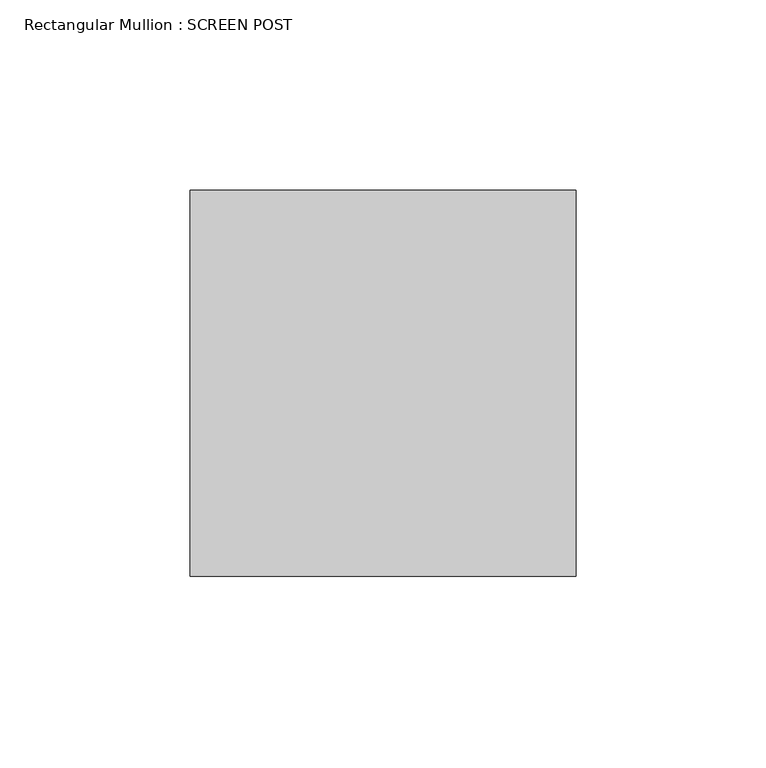
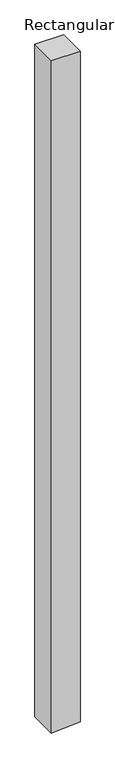
"""IFC4 building model written with IfcOpenShell, lengths in millimetres: member geometry, Rectangular Mullion : SCREEN POST."""

from ifc_helpers import new_model, si_unit, frame, origin, place, context, project, spatial, polyline, outline, extrude, source, transform, mapped, element, save


def rectangular_mullion_screen_post_f0368bff(model_context):
    return source(origin(), model_context, "Body", "SweptSolid", [
        extrude(outline(polyline([(0.0, 50.8), (0.0, -50.8), (-2524.2283574, -50.8), (-2521.4451532, -6.3490391), (-2517.8668852, 50.8), (0.0, 50.8)])), frame((0.0, -50.8, 0.0), z_axis=(0.0, 1.0, 0.0), x_axis=(0.0, 0.0, 1.0)), (0.0, 0.0, 1.0), 101.6),
    ])


if __name__ == "__main__":
    model = new_model("IFC4")
    model_context = context("Model", 3, world=origin())
    ifc_project = project(units=[si_unit("LENGTHUNIT", "METRE", prefix="MILLI")], contexts=[model_context])
    site = spatial("IfcSite", under=ifc_project)
    building = spatial("IfcBuilding", under=site)
    placement = place(None, origin())
    rectangular_mullion_screen_post_shape = rectangular_mullion_screen_post_f0368bff(model_context)
    element("IfcMember", 1, ObjectType="Rectangular Mullion : SCREEN POST", at=placement, inside=building, context=model_context, shape_type="MappedRepresentation", body=[
        mapped(rectangular_mullion_screen_post_shape, transform((0.0, 0.0, 0.0), x_axis=(1.0, 0.0, 0.0), y_axis=(0.0, 1.0, 0.0), z_axis=(0.0, 0.0, 1.0))),
    ])
    save(model, "model.ifc")

# Revit data of these elements
# Type "Rectangular Mullion : SCREEN POST"
#   built-in parameter 1007304 = 0.333333 (stored number, unit not read)
#   built-in parameter 1007301 = 0.166667 (stored number, unit not read)
#   built-in parameter 1007300 = 0.166667 (stored number, unit not read)
# Element 1 (IfcMember, "Rectangular Mullion : SCREEN POST")
#   Materials on its faces: "SCREEN PORCH FRAMING"
# Materials
#   "SCREEN PORCH FRAMING": class "Wood", colour RGB 164 134 123, transparency 0, Description = "Pinus Echinata", Cost = 0
